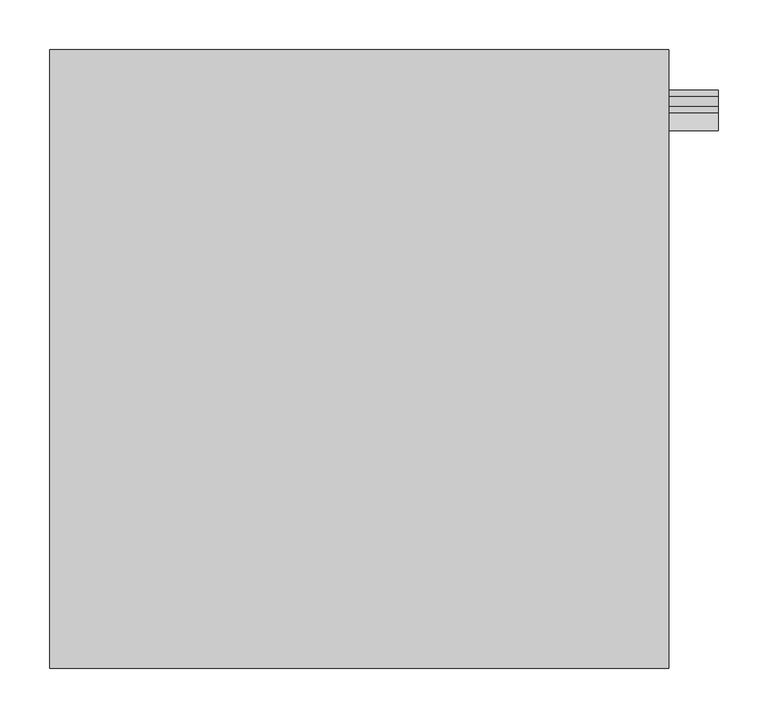
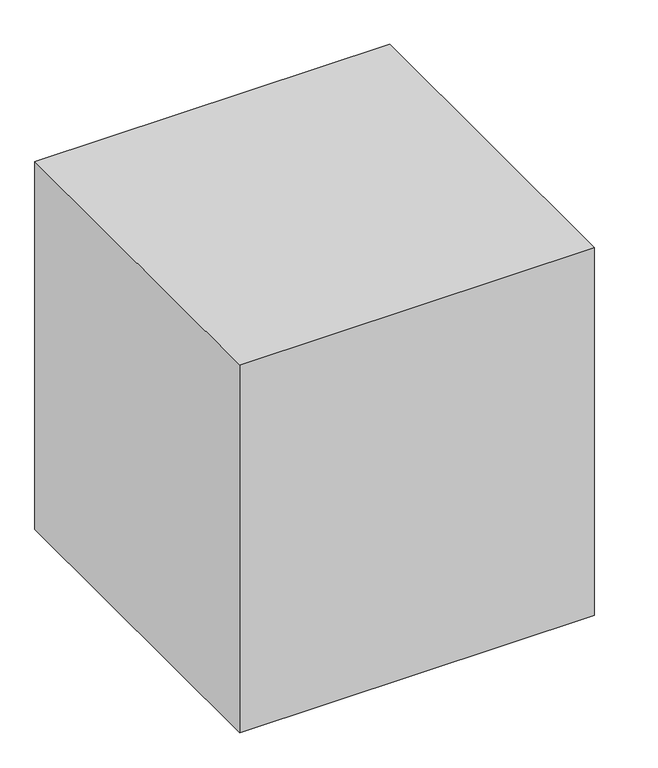
"""IFC4 building model written with IfcOpenShell, lengths in millimetres: proxy geometry, Evaporator coil : Evaporator coil."""

import ifcopenshell
import ifcopenshell.guid

model = None  # the IFC model being written
_history = None  # IfcOwnerHistory: only IFC2X3 demands one
_inside = {}  # id of a spatial element -> (the spatial element, [elements in it])
_under = {}  # id of a project, library or spatial element -> (it, [spatial elements below it])
_declared = {}  # id of a project -> (the project, [libraries it declares])
_typed = {}  # id of a type object -> (the type object, [elements of that type])
_made_of = {}  # id of a material, layer set ... -> (it, [elements and type objects made of it])


def new_model(schema):
    """Start an empty IFC model of exactly this schema.

    Asked for "IFC4X3", IfcOpenShell would pick the latest addendum, in which some entities
    have other attributes; the version numbers below select the first issue.
    IFC2X3 requires an IfcOwnerHistory on every rooted entity: one is made here for all.
    """
    global model, _history
    if schema == "IFC4X3":
        model = ifcopenshell.file(schema_version=(4, 3, 0, 0))
    else:
        model = ifcopenshell.file(schema=schema)
    _inside.clear()
    _under.clear()
    _declared.clear()
    _typed.clear()
    _made_of.clear()
    _history = None
    if model.schema == "IFC2X3":
        org = make("IfcOrganization", Name="unknown")
        user = make(
            "IfcPersonAndOrganization",
            ThePerson=make("IfcPerson", FamilyName="unknown"),
            TheOrganization=org,
        )
        app = make(
            "IfcApplication",
            ApplicationDeveloper=org,
            Version="unknown",
            ApplicationFullName="unknown",
            ApplicationIdentifier="unknown",
        )
        _history = make(
            "IfcOwnerHistory",
            OwningUser=user,
            OwningApplication=app,
            ChangeAction="ADDED",
            CreationDate=0,
        )
    return model


def make(cls, **values):
    """One entity of the class cls with the attributes given. An attribute that is None is left unset."""
    return model.create_entity(
        cls, **{name: value for name, value in values.items() if value is not None}
    )


def rooted(cls, **values):
    """An entity with a GlobalId (a new one), such as an element, a storey or a relation."""
    return make(cls, GlobalId=ifcopenshell.guid.new(), OwnerHistory=_history, **values)


def si_unit(unit_type, name, prefix=None):
    """IfcSIUnit, for example si_unit("LENGTHUNIT", "METRE", prefix="MILLI")."""
    return make("IfcSIUnit", UnitType=unit_type, Prefix=prefix, Name=name)


def assignment(units):
    """IfcUnitAssignment: the units of a project."""
    return None if units is None else make("IfcUnitAssignment", Units=units)


def point(xyz):
    """IfcCartesianPoint."""
    return None if xyz is None else make("IfcCartesianPoint", Coordinates=xyz)


def direction(xyz):
    """IfcDirection."""
    return None if xyz is None else make("IfcDirection", DirectionRatios=xyz)


def frame(location, z_axis=None, x_axis=None):
    """IfcAxis2Placement3D, a coordinate frame: its origin and axes. An axis left out is left unset."""
    return make(
        "IfcAxis2Placement3D",
        Location=point(location),
        Axis=direction(z_axis),
        RefDirection=direction(x_axis),
    )


def frame_2d(location, x_axis=None):
    """IfcAxis2Placement2D, a coordinate frame in the plane: its origin and x axis."""
    return make(
        "IfcAxis2Placement2D", Location=point(location), RefDirection=direction(x_axis)
    )


def origin():
    """The frame at (0, 0, 0) with its axes left unset."""
    return frame((0.0, 0.0, 0.0))


def origin_with_axes():
    """The frame at (0, 0, 0) with the z axis (0, 0, 1) and the x axis (1, 0, 0) written out."""
    return frame((0.0, 0.0, 0.0), z_axis=(0.0, 0.0, 1.0), x_axis=(1.0, 0.0, 0.0))


def place(relative_to, where):
    """IfcLocalPlacement: puts the frame where relative to a parent placement (None: the world)."""
    return make(
        "IfcLocalPlacement", PlacementRelTo=relative_to, RelativePlacement=where
    )


def context(
    kind, dimensions, precision=None, world=None, true_north=None, identifier=None
):
    """IfcGeometricRepresentationContext, for example the 3D "Model" context."""
    return make(
        "IfcGeometricRepresentationContext",
        ContextIdentifier=identifier,
        ContextType=kind,
        CoordinateSpaceDimension=dimensions,
        Precision=precision,
        WorldCoordinateSystem=world,
        TrueNorth=true_north,
    )


def project(units=None, contexts=None):
    """IfcProject with its units and contexts."""
    return rooted(
        "IfcProject",
        Name="project",
        RepresentationContexts=contexts,
        UnitsInContext=assignment(units),
    )


def spatial(cls, under=None, at=None, **own):
    """A site, building, storey or space (cls), placed at a placement, below another one or the project."""
    s = rooted(cls, ObjectPlacement=at, **own)
    if under is not None:
        _under.setdefault(under.id(), (under, []))[1].append(s)
    return s


def polyline(points):
    """IfcPolyline through the points."""
    return make("IfcPolyline", Points=[point(p) for p in points])


def circle_curve(where, radius):
    """IfcCircle in the frame where."""
    return make("IfcCircle", Position=where, Radius=radius)


def trimmed(basis, trim1, trim2, sense, master):
    """IfcTrimmedCurve: the piece of a basis curve between two trims."""
    return make(
        "IfcTrimmedCurve",
        BasisCurve=basis,
        Trim1=trim1,
        Trim2=trim2,
        SenseAgreement=sense,
        MasterRepresentation=master,
    )


def segment(curve, same_sense, transition):
    """IfcCompositeCurveSegment."""
    return make(
        "IfcCompositeCurveSegment",
        Transition=transition,
        SameSense=same_sense,
        ParentCurve=curve,
    )


def composite_curve(segments, self_intersect=None):
    """IfcCompositeCurve: segments joined end to end."""
    return make("IfcCompositeCurve", Segments=segments, SelfIntersect=self_intersect)


def outline(outer, holes=None, kind="AREA"):
    """IfcArbitraryClosedProfileDef: a profile drawn as a closed curve; with holes, ...WithVoids."""
    if holes is None:
        return make("IfcArbitraryClosedProfileDef", ProfileType=kind, OuterCurve=outer)
    return make(
        "IfcArbitraryProfileDefWithVoids",
        ProfileType=kind,
        OuterCurve=outer,
        InnerCurves=holes,
    )


def extrude(swept, where, along, depth):
    """IfcExtrudedAreaSolid: the profile swept, set in the frame where, extruded along a direction by depth."""
    return make(
        "IfcExtrudedAreaSolid",
        SweptArea=swept,
        Position=where,
        ExtrudedDirection=direction(along),
        Depth=depth,
    )


def shape(context_of_items, identifier, shape_type, items):
    """IfcShapeRepresentation: the items that make up one representation, for example the "Body"."""
    return make(
        "IfcShapeRepresentation",
        ContextOfItems=context_of_items,
        RepresentationIdentifier=identifier,
        RepresentationType=shape_type,
        Items=items,
    )


def source(mapping_origin, context_of_items, identifier, shape_type, items):
    """IfcRepresentationMap: a shape defined once, which mapped items show again and again."""
    return make(
        "IfcRepresentationMap",
        MappingOrigin=mapping_origin,
        MappedRepresentation=shape(context_of_items, identifier, shape_type, items),
    )


def transform(
    local_origin,
    x_axis=None,
    y_axis=None,
    z_axis=None,
    scale=None,
    scale2=None,
    scale3=None,
    uniform=True,
):
    """IfcCartesianTransformationOperator3D, or its non-uniform kind. x_axis, y_axis, z_axis: its Axis1, 2, 3."""
    if uniform:
        return make(
            "IfcCartesianTransformationOperator3D",
            Axis1=direction(x_axis),
            Axis2=direction(y_axis),
            LocalOrigin=point(local_origin),
            Scale=scale,
            Axis3=direction(z_axis),
        )
    return make(
        "IfcCartesianTransformationOperator3DnonUniform",
        Axis1=direction(x_axis),
        Axis2=direction(y_axis),
        LocalOrigin=point(local_origin),
        Scale=scale,
        Axis3=direction(z_axis),
        Scale2=scale2,
        Scale3=scale3,
    )


def mapped(mapping_source, mapping_target):
    """IfcMappedItem: shows the shape of a source again, moved by a transform."""
    return make(
        "IfcMappedItem", MappingSource=mapping_source, MappingTarget=mapping_target
    )


def made_of(thing, what):
    """Note that an element or type object is made of a material, layer set ...; save() writes the relation."""
    if what is not None:
        _made_of.setdefault(what.id(), (what, []))[1].append(thing)
    return thing


def element(
    cls,
    number,
    at=None,
    inside=None,
    cuts=None,
    type_object=None,
    material=None,
    context=None,
    identifier="Body",
    shape_type=None,
    held_by="IfcProductDefinitionShape",
    body=None,
    shapes=None,
    **own,
):
    """One element of the class cls, such as IfcWall. Its Tag is "e" and its number.

    at: its placement. inside: the storey or other place that contains it. cuts: it is an
    opening in that element (IfcRelVoidsElement). A single representation is given by context,
    identifier, shape_type and body (its items); several are given by shapes. held_by: the class
    of the entity that holds the representations. save() writes the other relations.
    """
    e = rooted(cls, Tag="e%d" % number, ObjectPlacement=at, **own)
    if body is not None:
        shapes = [shape(context, identifier, shape_type, body)]
    if shapes is not None:
        e.Representation = make(held_by, Representations=shapes)
    if inside is not None:
        _inside.setdefault(inside.id(), (inside, []))[1].append(e)
    if cuts is not None:
        rooted(
            "IfcRelVoidsElement", RelatingBuildingElement=cuts, RelatedOpeningElement=e
        )
    if type_object is not None:
        _typed.setdefault(type_object.id(), (type_object, []))[1].append(e)
    return made_of(e, material)


def aggregate(whole, parts):
    """IfcRelAggregates: a whole, such as a stair, and the parts it consists of."""
    return rooted("IfcRelAggregates", RelatingObject=whole, RelatedObjects=parts)


def save(model, path):
    """Write the relations noted so far, then the file.

    IfcRelAggregates (storeys below a building ...), IfcRelContainedInSpatialStructure (elements
    in a storey), IfcRelDefinesByType, IfcRelAssociatesMaterial and IfcRelDeclares: one each for
    every whole, place, type object, material and project.
    """
    for whole, parts in _under.values():
        aggregate(whole, parts)
    for where, things in _inside.values():
        rooted(
            "IfcRelContainedInSpatialStructure",
            RelatedElements=things,
            RelatingStructure=where,
        )
    for kind, things in _typed.values():
        rooted("IfcRelDefinesByType", RelatedObjects=things, RelatingType=kind)
    for what, things in _made_of.values():
        rooted("IfcRelAssociatesMaterial", RelatedObjects=things, RelatingMaterial=what)
    for by, libraries in _declared.values():
        rooted("IfcRelDeclares", RelatingContext=by, RelatedDefinitions=libraries)
    model.write(path)


def mechanical_equipment_1ffd6ebc(model_context):
    return source(origin(), model_context, "Body", "SweptSolid", [
        extrude(outline(composite_curve([segment(trimmed(circle_curve(frame_2d((259.15, 455.6)), 4.8), [point((254.35, 455.6))], [point((263.95, 455.6))], False, "CARTESIAN"), True, "CONTINUOUS"), segment(trimmed(circle_curve(frame_2d((259.15, 455.6)), 4.8), [point((263.95, 455.6))], [point((254.35, 455.6))], False, "CARTESIAN"), True, "CONTINUOUS")], self_intersect=False)), frame((311.15, 0.0, 0.0), z_axis=(1.0, 0.0, 0.0), x_axis=(0.0, 1.0, 0.0)), (0.0, 0.0, 1.0), 50.0),
        extrude(outline(composite_curve([segment(trimmed(circle_curve(frame_2d((259.15, 365.6)), 11.1), [point((248.05, 365.6))], [point((270.25, 365.6))], False, "CARTESIAN"), True, "CONTINUOUS"), segment(trimmed(circle_curve(frame_2d((259.15, 365.6)), 11.1), [point((270.25, 365.6))], [point((248.05, 365.6))], False, "CARTESIAN"), True, "CONTINUOUS")], self_intersect=False)), frame((311.15, 0.0, 0.0), z_axis=(1.0, 0.0, 0.0), x_axis=(0.0, 1.0, 0.0)), (0.0, 0.0, 1.0), 50.0),
        extrude(outline(composite_curve([segment(trimmed(circle_curve(frame_2d((239.15, 35.0)), 9.5), [point((229.65, 35.0))], [point((248.65, 35.0))], False, "CARTESIAN"), True, "CONTINUOUS"), segment(trimmed(circle_curve(frame_2d((239.15, 35.0)), 9.5), [point((248.65, 35.0))], [point((229.65, 35.0))], False, "CARTESIAN"), True, "CONTINUOUS")], self_intersect=False)), frame((311.15, 0.0, 0.0), z_axis=(1.0, 0.0, 0.0), x_axis=(0.0, 1.0, 0.0)), (0.0, 0.0, 1.0), 50.0),
        extrude(outline(polyline([(311.15, 311.15), (311.15, -311.15), (-311.15, -311.15), (-311.15, 311.15), (311.15, 311.15)])), origin_with_axes(), (0.0, 0.0, 1.0), 682.6),
    ])


if __name__ == "__main__":
    model = new_model("IFC4")
    model_context = context("Model", 3, world=origin())
    ifc_project = project(units=[si_unit("LENGTHUNIT", "METRE", prefix="MILLI")], contexts=[model_context])
    site = spatial("IfcSite", under=ifc_project)
    building = spatial("IfcBuilding", under=site)
    placement = place(None, origin())
    mechanical_equipment_shape = mechanical_equipment_1ffd6ebc(model_context)
    element("IfcBuildingElementProxy", 1, Name="Evaporator coil : Evaporator coil", ObjectType="Evaporator coil : Evaporator coil", at=placement, inside=building, context=model_context, shape_type="MappedRepresentation", body=[
        mapped(mechanical_equipment_shape, transform((0.0, 0.0, 0.0), x_axis=(1.0, 0.0, 0.0), y_axis=(0.0, 1.0, 0.0), z_axis=(0.0, 0.0, 1.0))),
    ])
    save(model, "model.ifc")

# Revit data of these elements
# Type "Evaporator coil : Evaporator coil"
#   Type Mark = "EVC-01"
#   Refrigerent = "R410"
#   Width = 622.3 mm
#   Suction line size = 22.2 mm
#   Length = 622.3 mm
#   Height = 682.6 mm
#   Drain Dia = 19 mm
#   Coil pressure drop = 0.00 in-wg
